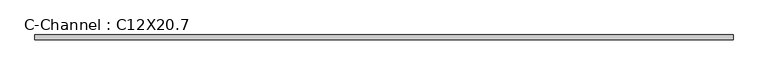
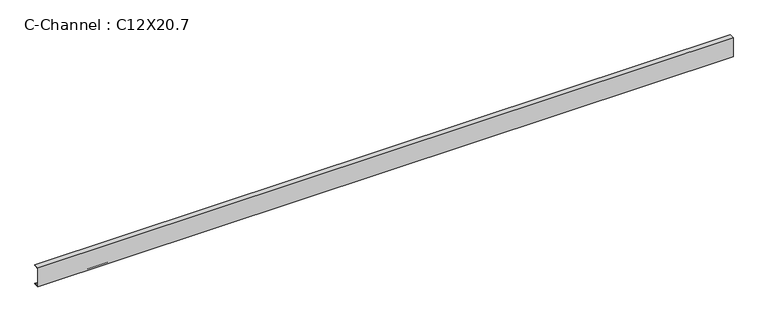
"""IFC4 building model written with IfcOpenShell, lengths in millimetres: beam geometry, C-Channel : C12X20.7."""

from ifc_helpers import new_model, si_unit, point, frame, frame_2d, origin, place, context, project, spatial, polyline, circle_curve, trimmed, segment, composite_curve, outline, extrude, source, transform, mapped, element, save


def c_channel_c12x20_7_457acdaa(model_context):
    return source(origin(), model_context, "Body", "SweptSolid", [
        extrude(outline(composite_curve([segment(polyline([(-17.7292, 152.4), (56.9468, 152.4)]), True, "CONTINUOUS"), segment(trimmed(circle_curve(frame_2d((44.2214, 152.4)), 12.7254), [point((56.9468, 152.4))], [point((44.2214, 139.6746))], False, "CARTESIAN"), True, "CONTINUOUS"), segment(polyline([(44.2214, 139.6746), (-10.5664, 130.997065), (-10.5664, -130.997065), (44.2214, -139.6746)]), True, "CONTINUOUS"), segment(trimmed(circle_curve(frame_2d((44.2214, -152.4)), 12.7254), [point((44.2214, -139.6746))], [point((56.9468, -152.4))], False, "CARTESIAN"), True, "CONTINUOUS"), segment(polyline([(56.9468, -152.4), (-17.7292, -152.4), (-17.7292, 152.4)]), True, "CONTINUOUS")], self_intersect=False)), frame((-5185.9694787, 0.0, 0.0), z_axis=(1.0, 0.0, 0.0), x_axis=(0.0, 1.0, 0.0)), (0.0, 0.0, 1.0), 10455.1373218),
    ])


if __name__ == "__main__":
    model = new_model("IFC4")
    model_context = context("Model", 3, world=origin())
    ifc_project = project(units=[si_unit("LENGTHUNIT", "METRE", prefix="MILLI")], contexts=[model_context])
    site = spatial("IfcSite", under=ifc_project)
    building = spatial("IfcBuilding", under=site)
    placement = place(None, origin())
    c_channel_c12x20_7_shape = c_channel_c12x20_7_457acdaa(model_context)
    element("IfcBeam", 1, ObjectType="C-Channel : C12X20.7", at=placement, inside=building, context=model_context, shape_type="MappedRepresentation", body=[
        mapped(c_channel_c12x20_7_shape, transform((0.0, 0.0, 0.0), x_axis=(1.0, 0.0, 0.0), y_axis=(0.0, 1.0, 0.0), z_axis=(0.0, 0.0, 1.0))),
    ])
    save(model, "model.ifc")

# Revit data of these elements
# Type "C-Channel : C12X20.7"
#   Assembly Code = "B10"
#   W = 20.7
#   Start Extension Calculation [instance default] = 10' - 0"
#   Start Extension [instance default] = -0' - 0 1/2"
#   End Extension Calculation [instance default] = 10' - 0"
#   End Extension [instance default] = -0' - 0 1/2"
#   Length [instance default] = 5' - 0"
#   bf = 0' - 2.94"
#   d = 1' - 0"
#   tf = 0' - 0.501"
#   tw = 0' - 0.282"
#   x = 0' - 0.698"
#   A = 0.0422222 SF
#   Structural Material [instance default] = Metal - Steel - ASTM A36
# Element 1 (IfcBeam, "C-Channel : C12X20.7")
#   Materials on its faces: "Metal - Steel - ASTM A36"
# Materials
#   "Metal - Steel - ASTM A36": class "Metal", colour RGB 199 199 199, transparency 0
